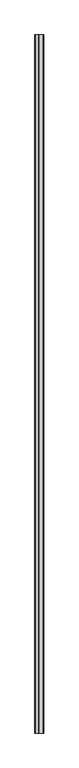
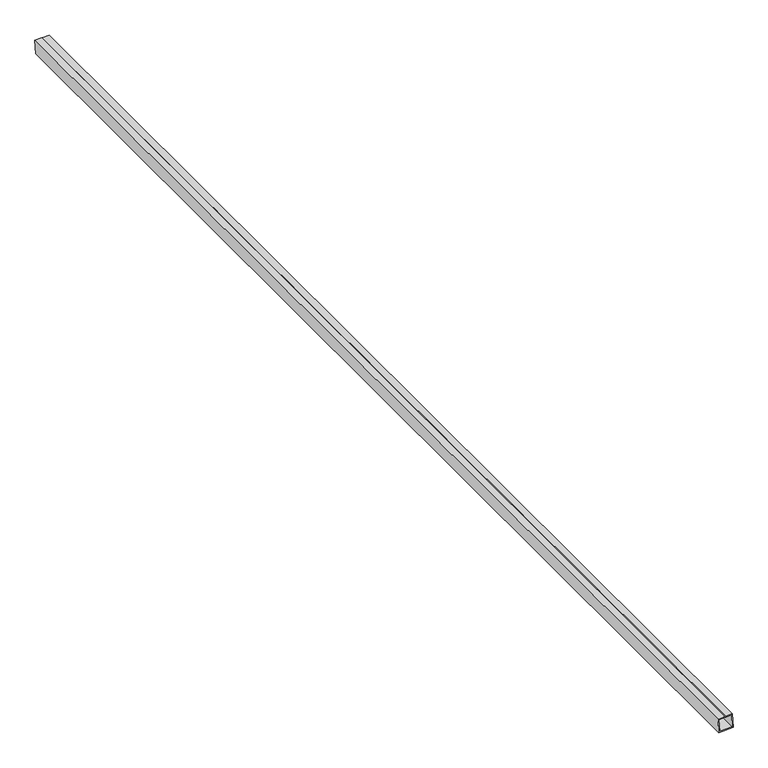
"""IFC4 building model written with IfcOpenShell, lengths in millimetres: proxy geometry, Inner panel:Inner panel:1:Inner panel:1 : Inner panel:Inner panel:300324:2:Inner panel:1:Inner panel:1 : Inner panel:Inner panel:300324:2 : Inner panel:Inner panel:1:Inner panel:1 : Inner panel:Inner panel:300324:300043:33 : Inner panel:Inner panel:1:Inner panel:1 : Inner panel:Inner panel:300324:2:Inner panel:1:Inner panel:1 : Inner panel:Inner panel:300324:2 : Inner panel:Inner panel:1:Inner panel:1 : Inner panel:Inner panel:300324:300043:308120."""

import ifcopenshell
import ifcopenshell.guid

model = None  # the IFC model being written
_history = None  # IfcOwnerHistory: only IFC2X3 demands one
_inside = {}  # id of a spatial element -> (the spatial element, [elements in it])
_under = {}  # id of a project, library or spatial element -> (it, [spatial elements below it])
_declared = {}  # id of a project -> (the project, [libraries it declares])
_typed = {}  # id of a type object -> (the type object, [elements of that type])
_made_of = {}  # id of a material, layer set ... -> (it, [elements and type objects made of it])


def new_model(schema):
    """Start an empty IFC model of exactly this schema.

    Asked for "IFC4X3", IfcOpenShell would pick the latest addendum, in which some entities
    have other attributes; the version numbers below select the first issue.
    IFC2X3 requires an IfcOwnerHistory on every rooted entity: one is made here for all.
    """
    global model, _history
    if schema == "IFC4X3":
        model = ifcopenshell.file(schema_version=(4, 3, 0, 0))
    else:
        model = ifcopenshell.file(schema=schema)
    _inside.clear()
    _under.clear()
    _declared.clear()
    _typed.clear()
    _made_of.clear()
    _history = None
    if model.schema == "IFC2X3":
        org = make("IfcOrganization", Name="unknown")
        user = make(
            "IfcPersonAndOrganization",
            ThePerson=make("IfcPerson", FamilyName="unknown"),
            TheOrganization=org,
        )
        app = make(
            "IfcApplication",
            ApplicationDeveloper=org,
            Version="unknown",
            ApplicationFullName="unknown",
            ApplicationIdentifier="unknown",
        )
        _history = make(
            "IfcOwnerHistory",
            OwningUser=user,
            OwningApplication=app,
            ChangeAction="ADDED",
            CreationDate=0,
        )
    return model


def make(cls, **values):
    """One entity of the class cls with the attributes given. An attribute that is None is left unset."""
    return model.create_entity(
        cls, **{name: value for name, value in values.items() if value is not None}
    )


def rooted(cls, **values):
    """An entity with a GlobalId (a new one), such as an element, a storey or a relation."""
    return make(cls, GlobalId=ifcopenshell.guid.new(), OwnerHistory=_history, **values)


def si_unit(unit_type, name, prefix=None):
    """IfcSIUnit, for example si_unit("LENGTHUNIT", "METRE", prefix="MILLI")."""
    return make("IfcSIUnit", UnitType=unit_type, Prefix=prefix, Name=name)


def assignment(units):
    """IfcUnitAssignment: the units of a project."""
    return None if units is None else make("IfcUnitAssignment", Units=units)


def point(xyz):
    """IfcCartesianPoint."""
    return None if xyz is None else make("IfcCartesianPoint", Coordinates=xyz)


def direction(xyz):
    """IfcDirection."""
    return None if xyz is None else make("IfcDirection", DirectionRatios=xyz)


def frame(location, z_axis=None, x_axis=None):
    """IfcAxis2Placement3D, a coordinate frame: its origin and axes. An axis left out is left unset."""
    return make(
        "IfcAxis2Placement3D",
        Location=point(location),
        Axis=direction(z_axis),
        RefDirection=direction(x_axis),
    )


def origin():
    """The frame at (0, 0, 0) with its axes left unset."""
    return frame((0.0, 0.0, 0.0))


def place(relative_to, where):
    """IfcLocalPlacement: puts the frame where relative to a parent placement (None: the world)."""
    return make(
        "IfcLocalPlacement", PlacementRelTo=relative_to, RelativePlacement=where
    )


def context(
    kind, dimensions, precision=None, world=None, true_north=None, identifier=None
):
    """IfcGeometricRepresentationContext, for example the 3D "Model" context."""
    return make(
        "IfcGeometricRepresentationContext",
        ContextIdentifier=identifier,
        ContextType=kind,
        CoordinateSpaceDimension=dimensions,
        Precision=precision,
        WorldCoordinateSystem=world,
        TrueNorth=true_north,
    )


def project(units=None, contexts=None):
    """IfcProject with its units and contexts."""
    return rooted(
        "IfcProject",
        Name="project",
        RepresentationContexts=contexts,
        UnitsInContext=assignment(units),
    )


def spatial(cls, under=None, at=None, **own):
    """A site, building, storey or space (cls), placed at a placement, below another one or the project."""
    s = rooted(cls, ObjectPlacement=at, **own)
    if under is not None:
        _under.setdefault(under.id(), (under, []))[1].append(s)
    return s


def polyline(points):
    """IfcPolyline through the points."""
    return make("IfcPolyline", Points=[point(p) for p in points])


def outline(outer, holes=None, kind="AREA"):
    """IfcArbitraryClosedProfileDef: a profile drawn as a closed curve; with holes, ...WithVoids."""
    if holes is None:
        return make("IfcArbitraryClosedProfileDef", ProfileType=kind, OuterCurve=outer)
    return make(
        "IfcArbitraryProfileDefWithVoids",
        ProfileType=kind,
        OuterCurve=outer,
        InnerCurves=holes,
    )


def extrude(swept, where, along, depth):
    """IfcExtrudedAreaSolid: the profile swept, set in the frame where, extruded along a direction by depth."""
    return make(
        "IfcExtrudedAreaSolid",
        SweptArea=swept,
        Position=where,
        ExtrudedDirection=direction(along),
        Depth=depth,
    )


def shape(context_of_items, identifier, shape_type, items):
    """IfcShapeRepresentation: the items that make up one representation, for example the "Body"."""
    return make(
        "IfcShapeRepresentation",
        ContextOfItems=context_of_items,
        RepresentationIdentifier=identifier,
        RepresentationType=shape_type,
        Items=items,
    )


def source(mapping_origin, context_of_items, identifier, shape_type, items):
    """IfcRepresentationMap: a shape defined once, which mapped items show again and again."""
    return make(
        "IfcRepresentationMap",
        MappingOrigin=mapping_origin,
        MappedRepresentation=shape(context_of_items, identifier, shape_type, items),
    )


def transform(
    local_origin,
    x_axis=None,
    y_axis=None,
    z_axis=None,
    scale=None,
    scale2=None,
    scale3=None,
    uniform=True,
):
    """IfcCartesianTransformationOperator3D, or its non-uniform kind. x_axis, y_axis, z_axis: its Axis1, 2, 3."""
    if uniform:
        return make(
            "IfcCartesianTransformationOperator3D",
            Axis1=direction(x_axis),
            Axis2=direction(y_axis),
            LocalOrigin=point(local_origin),
            Scale=scale,
            Axis3=direction(z_axis),
        )
    return make(
        "IfcCartesianTransformationOperator3DnonUniform",
        Axis1=direction(x_axis),
        Axis2=direction(y_axis),
        LocalOrigin=point(local_origin),
        Scale=scale,
        Axis3=direction(z_axis),
        Scale2=scale2,
        Scale3=scale3,
    )


def mapped(mapping_source, mapping_target):
    """IfcMappedItem: shows the shape of a source again, moved by a transform."""
    return make(
        "IfcMappedItem", MappingSource=mapping_source, MappingTarget=mapping_target
    )


def made_of(thing, what):
    """Note that an element or type object is made of a material, layer set ...; save() writes the relation."""
    if what is not None:
        _made_of.setdefault(what.id(), (what, []))[1].append(thing)
    return thing


def element(
    cls,
    number,
    at=None,
    inside=None,
    cuts=None,
    type_object=None,
    material=None,
    context=None,
    identifier="Body",
    shape_type=None,
    held_by="IfcProductDefinitionShape",
    body=None,
    shapes=None,
    **own,
):
    """One element of the class cls, such as IfcWall. Its Tag is "e" and its number.

    at: its placement. inside: the storey or other place that contains it. cuts: it is an
    opening in that element (IfcRelVoidsElement). A single representation is given by context,
    identifier, shape_type and body (its items); several are given by shapes. held_by: the class
    of the entity that holds the representations. save() writes the other relations.
    """
    e = rooted(cls, Tag="e%d" % number, ObjectPlacement=at, **own)
    if body is not None:
        shapes = [shape(context, identifier, shape_type, body)]
    if shapes is not None:
        e.Representation = make(held_by, Representations=shapes)
    if inside is not None:
        _inside.setdefault(inside.id(), (inside, []))[1].append(e)
    if cuts is not None:
        rooted(
            "IfcRelVoidsElement", RelatingBuildingElement=cuts, RelatedOpeningElement=e
        )
    if type_object is not None:
        _typed.setdefault(type_object.id(), (type_object, []))[1].append(e)
    return made_of(e, material)


def aggregate(whole, parts):
    """IfcRelAggregates: a whole, such as a stair, and the parts it consists of."""
    return rooted("IfcRelAggregates", RelatingObject=whole, RelatedObjects=parts)


def save(model, path):
    """Write the relations noted so far, then the file.

    IfcRelAggregates (storeys below a building ...), IfcRelContainedInSpatialStructure (elements
    in a storey), IfcRelDefinesByType, IfcRelAssociatesMaterial and IfcRelDeclares: one each for
    every whole, place, type object, material and project.
    """
    for whole, parts in _under.values():
        aggregate(whole, parts)
    for where, things in _inside.values():
        rooted(
            "IfcRelContainedInSpatialStructure",
            RelatedElements=things,
            RelatingStructure=where,
        )
    for kind, things in _typed.values():
        rooted("IfcRelDefinesByType", RelatedObjects=things, RelatingType=kind)
    for what, things in _made_of.values():
        rooted("IfcRelAssociatesMaterial", RelatedObjects=things, RelatingMaterial=what)
    for by, libraries in _declared.values():
        rooted("IfcRelDeclares", RelatingContext=by, RelatedDefinitions=libraries)
    model.write(path)


def generic_models_ba9b2a3c(model_context):
    return source(origin(), model_context, "Body", "SweptSolid", [
        extrude(outline(polyline([(4022.4868814, 562107.7864431), (4020.1076958, 562107.8855758), (4020.7685807, 562123.7468134), (3987.4599819, 562125.1346716), (3986.0721236, 562091.8260728), (4019.3807224, 562090.4382145), (4020.0416073, 562106.2994521), (4022.420793, 562106.2003193), (4021.6607753, 562087.9598962), (3983.5938052, 562089.5460199), (3985.179929, 562127.61299), (4023.2468991, 562126.0268663), (4022.4868814, 562107.7864431)])), frame((0.0, -578797.4913841, 0.0), z_axis=(0.0, 1.0, 0.0), x_axis=(0.0, 0.0, 1.0)), (0.0, 0.0, 1.0), 3121.0250001),
    ])


if __name__ == "__main__":
    model = new_model("IFC4")
    model_context = context("Model", 3, world=origin())
    ifc_project = project(units=[si_unit("LENGTHUNIT", "METRE", prefix="MILLI")], contexts=[model_context])
    site = spatial("IfcSite", under=ifc_project)
    building = spatial("IfcBuilding", under=site)
    placement = place(None, origin())
    generic_models_shape = generic_models_ba9b2a3c(model_context)
    element("IfcBuildingElementProxy", 1, Name="Inner panel:Inner panel:1:Inner panel:1 : Inner panel:Inner panel:300324:2:Inner panel:1:Inner panel:1 : Inner panel:Inner panel:300324:2 : Inner panel:Inner panel:1:Inner panel:1 : Inner panel:Inner panel:300324:300043:33 : Inner panel:Inner panel:1:Inner panel:1 : Inner panel:Inner panel:300324:2:Inner panel:1:Inner panel:1 : Inner panel:Inner panel:300324:2 : Inner panel:Inner panel:1:Inner panel:1 : Inner panel:Inner panel:300324:300043:308120", ObjectType="Inner panel:Inner panel:1:Inner panel:1 : Inner panel:Inner panel:300324:2:Inner panel:1:Inner panel:1 : Inner panel:Inner panel:300324:2 : Inner panel:Inner panel:1:Inner panel:1 : Inner panel:Inner panel:300324:300043:33 : Inner panel:Inner panel:1:Inner panel:1 : Inner panel:Inner panel:300324:2:Inner panel:1:Inner panel:1 : Inner panel:Inner panel:300324:2 : Inner panel:Inner panel:1:Inner panel:1 : Inner panel:Inner panel:300324:300043:308120", at=placement, inside=building, context=model_context, shape_type="MappedRepresentation", body=[
        mapped(generic_models_shape, transform((0.0, 0.0, 0.0), x_axis=(1.0, 0.0, 0.0), y_axis=(0.0, 1.0, 0.0), z_axis=(0.0, 0.0, 1.0))),
    ])
    save(model, "model.ifc")

# Revit data of these elements
# Type "Inner panel:Inner panel:1:Inner panel:1 : Inner panel:Inner panel:300324:2:Inner panel:1:Inner panel:1 : Inner panel:Inner panel:300324:2 : Inner panel:Inner panel:1:Inner panel:1 : Inner panel:Inner panel:300324:300043:33 : Inner panel:Inner panel:1:Inner panel:1 : Inner panel:Inner panel:300324:2:Inner panel:1:Inner panel:1 : Inner panel:Inner panel:300324:2 : Inner panel:Inner panel:1:Inner panel:1 : Inner panel:Inner panel:300324:300043:308120"
#   NameOverride = "Inner panel:Inner panel:1:Inner panel:1 : Inner panel:Inner panel:300324:2:Inner panel:1:Inner panel:1 : Inner panel:Inner panel:300324:2 : Inner panel:Inner panel:1:Inner panel:1 : Inner panel:Inner panel:300324:300043:308120"
#   ObjectTypeOverride = "Inner panel:1:Inner panel:1 : Inner panel:Inner panel:300324:2 : Inner panel:Inner panel:1:Inner panel:1 : Inner panel:Inner panel:300324:300043"
#   Reference = "Inner panel"
#   Tag = "308120"
# Element 1 (IfcBuildingElementProxy, "Inner panel:Inner panel:1:Inner panel:1 : Inner panel:Inner panel:300324:2:Inner panel:1:Inner panel:1 : Inner panel:Inner panel:300324:2 : Inner panel:Inner panel:1:Inner panel:1 : Inner panel:Inner panel:300324:300043:33 : Inner panel:Inner panel:1:Inner panel:1 : Inner panel:Inner panel:300324:2:Inner panel:1:Inner panel:1 : Inner panel:Inner panel:300324:2 : Inner panel:Inner panel:1:Inner panel:1 : Inner panel:Inner panel:300324:300043:308120")
#   Materials on its faces: "1 1/2\" X 1 1/2\" x 1/8\" ALUM. TUBE (6061-T6) - (2) #16 WOOD SCREWS WITH 2.5\" EMBED AT EACH GLULAM - (1) SCREW AT ENDS"
# Materials
#   "1 1/2\" X 1 1/2\" x 1/8\" ALUM. TUBE (6061-T6) - (2) #16 WOOD SCREWS WITH 2.5\" EMBED AT EACH GLULAM - (1) SCREW AT ENDS": class "Unassigned", colour RGB 202 201 200, transparency 0, Cost = 0
